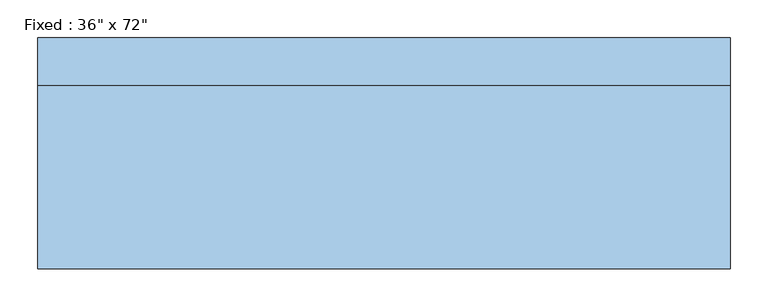
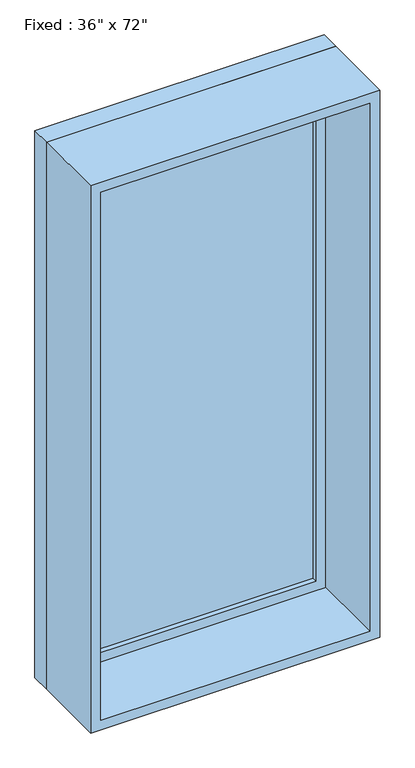
"""IFC4 building model written with IfcOpenShell, lengths in millimetres: window geometry."""

import ifcopenshell
import ifcopenshell.guid

model = None  # the IFC model being written
_history = None  # IfcOwnerHistory: only IFC2X3 demands one
_inside = {}  # id of a spatial element -> (the spatial element, [elements in it])
_under = {}  # id of a project, library or spatial element -> (it, [spatial elements below it])
_declared = {}  # id of a project -> (the project, [libraries it declares])
_typed = {}  # id of a type object -> (the type object, [elements of that type])
_made_of = {}  # id of a material, layer set ... -> (it, [elements and type objects made of it])


def new_model(schema):
    """Start an empty IFC model of exactly this schema.

    Asked for "IFC4X3", IfcOpenShell would pick the latest addendum, in which some entities
    have other attributes; the version numbers below select the first issue.
    IFC2X3 requires an IfcOwnerHistory on every rooted entity: one is made here for all.
    """
    global model, _history
    if schema == "IFC4X3":
        model = ifcopenshell.file(schema_version=(4, 3, 0, 0))
    else:
        model = ifcopenshell.file(schema=schema)
    _inside.clear()
    _under.clear()
    _declared.clear()
    _typed.clear()
    _made_of.clear()
    _history = None
    if model.schema == "IFC2X3":
        org = make("IfcOrganization", Name="unknown")
        user = make(
            "IfcPersonAndOrganization",
            ThePerson=make("IfcPerson", FamilyName="unknown"),
            TheOrganization=org,
        )
        app = make(
            "IfcApplication",
            ApplicationDeveloper=org,
            Version="unknown",
            ApplicationFullName="unknown",
            ApplicationIdentifier="unknown",
        )
        _history = make(
            "IfcOwnerHistory",
            OwningUser=user,
            OwningApplication=app,
            ChangeAction="ADDED",
            CreationDate=0,
        )
    return model


def make(cls, **values):
    """One entity of the class cls with the attributes given. An attribute that is None is left unset."""
    return model.create_entity(
        cls, **{name: value for name, value in values.items() if value is not None}
    )


def rooted(cls, **values):
    """An entity with a GlobalId (a new one), such as an element, a storey or a relation."""
    return make(cls, GlobalId=ifcopenshell.guid.new(), OwnerHistory=_history, **values)


def si_unit(unit_type, name, prefix=None):
    """IfcSIUnit, for example si_unit("LENGTHUNIT", "METRE", prefix="MILLI")."""
    return make("IfcSIUnit", UnitType=unit_type, Prefix=prefix, Name=name)


def assignment(units):
    """IfcUnitAssignment: the units of a project."""
    return None if units is None else make("IfcUnitAssignment", Units=units)


def point(xyz):
    """IfcCartesianPoint."""
    return None if xyz is None else make("IfcCartesianPoint", Coordinates=xyz)


def direction(xyz):
    """IfcDirection."""
    return None if xyz is None else make("IfcDirection", DirectionRatios=xyz)


def frame(location, z_axis=None, x_axis=None):
    """IfcAxis2Placement3D, a coordinate frame: its origin and axes. An axis left out is left unset."""
    return make(
        "IfcAxis2Placement3D",
        Location=point(location),
        Axis=direction(z_axis),
        RefDirection=direction(x_axis),
    )


def origin():
    """The frame at (0, 0, 0) with its axes left unset."""
    return frame((0.0, 0.0, 0.0))


def place(relative_to, where):
    """IfcLocalPlacement: puts the frame where relative to a parent placement (None: the world)."""
    return make(
        "IfcLocalPlacement", PlacementRelTo=relative_to, RelativePlacement=where
    )


def context(
    kind, dimensions, precision=None, world=None, true_north=None, identifier=None
):
    """IfcGeometricRepresentationContext, for example the 3D "Model" context."""
    return make(
        "IfcGeometricRepresentationContext",
        ContextIdentifier=identifier,
        ContextType=kind,
        CoordinateSpaceDimension=dimensions,
        Precision=precision,
        WorldCoordinateSystem=world,
        TrueNorth=true_north,
    )


def project(units=None, contexts=None):
    """IfcProject with its units and contexts."""
    return rooted(
        "IfcProject",
        Name="project",
        RepresentationContexts=contexts,
        UnitsInContext=assignment(units),
    )


def spatial(cls, under=None, at=None, **own):
    """A site, building, storey or space (cls), placed at a placement, below another one or the project."""
    s = rooted(cls, ObjectPlacement=at, **own)
    if under is not None:
        _under.setdefault(under.id(), (under, []))[1].append(s)
    return s


def polyline(points):
    """IfcPolyline through the points."""
    return make("IfcPolyline", Points=[point(p) for p in points])


def outline(outer, holes=None, kind="AREA"):
    """IfcArbitraryClosedProfileDef: a profile drawn as a closed curve; with holes, ...WithVoids."""
    if holes is None:
        return make("IfcArbitraryClosedProfileDef", ProfileType=kind, OuterCurve=outer)
    return make(
        "IfcArbitraryProfileDefWithVoids",
        ProfileType=kind,
        OuterCurve=outer,
        InnerCurves=holes,
    )


def extrude(swept, where, along, depth):
    """IfcExtrudedAreaSolid: the profile swept, set in the frame where, extruded along a direction by depth."""
    return make(
        "IfcExtrudedAreaSolid",
        SweptArea=swept,
        Position=where,
        ExtrudedDirection=direction(along),
        Depth=depth,
    )


def shape(context_of_items, identifier, shape_type, items):
    """IfcShapeRepresentation: the items that make up one representation, for example the "Body"."""
    return make(
        "IfcShapeRepresentation",
        ContextOfItems=context_of_items,
        RepresentationIdentifier=identifier,
        RepresentationType=shape_type,
        Items=items,
    )


def source(mapping_origin, context_of_items, identifier, shape_type, items):
    """IfcRepresentationMap: a shape defined once, which mapped items show again and again."""
    return make(
        "IfcRepresentationMap",
        MappingOrigin=mapping_origin,
        MappedRepresentation=shape(context_of_items, identifier, shape_type, items),
    )


def transform(
    local_origin,
    x_axis=None,
    y_axis=None,
    z_axis=None,
    scale=None,
    scale2=None,
    scale3=None,
    uniform=True,
):
    """IfcCartesianTransformationOperator3D, or its non-uniform kind. x_axis, y_axis, z_axis: its Axis1, 2, 3."""
    if uniform:
        return make(
            "IfcCartesianTransformationOperator3D",
            Axis1=direction(x_axis),
            Axis2=direction(y_axis),
            LocalOrigin=point(local_origin),
            Scale=scale,
            Axis3=direction(z_axis),
        )
    return make(
        "IfcCartesianTransformationOperator3DnonUniform",
        Axis1=direction(x_axis),
        Axis2=direction(y_axis),
        LocalOrigin=point(local_origin),
        Scale=scale,
        Axis3=direction(z_axis),
        Scale2=scale2,
        Scale3=scale3,
    )


def mapped(mapping_source, mapping_target):
    """IfcMappedItem: shows the shape of a source again, moved by a transform."""
    return make(
        "IfcMappedItem", MappingSource=mapping_source, MappingTarget=mapping_target
    )


def made_of(thing, what):
    """Note that an element or type object is made of a material, layer set ...; save() writes the relation."""
    if what is not None:
        _made_of.setdefault(what.id(), (what, []))[1].append(thing)
    return thing


def element(
    cls,
    number,
    at=None,
    inside=None,
    cuts=None,
    type_object=None,
    material=None,
    context=None,
    identifier="Body",
    shape_type=None,
    held_by="IfcProductDefinitionShape",
    body=None,
    shapes=None,
    **own,
):
    """One element of the class cls, such as IfcWall. Its Tag is "e" and its number.

    at: its placement. inside: the storey or other place that contains it. cuts: it is an
    opening in that element (IfcRelVoidsElement). A single representation is given by context,
    identifier, shape_type and body (its items); several are given by shapes. held_by: the class
    of the entity that holds the representations. save() writes the other relations.
    """
    e = rooted(cls, Tag="e%d" % number, ObjectPlacement=at, **own)
    if body is not None:
        shapes = [shape(context, identifier, shape_type, body)]
    if shapes is not None:
        e.Representation = make(held_by, Representations=shapes)
    if inside is not None:
        _inside.setdefault(inside.id(), (inside, []))[1].append(e)
    if cuts is not None:
        rooted(
            "IfcRelVoidsElement", RelatingBuildingElement=cuts, RelatedOpeningElement=e
        )
    if type_object is not None:
        _typed.setdefault(type_object.id(), (type_object, []))[1].append(e)
    return made_of(e, material)


def aggregate(whole, parts):
    """IfcRelAggregates: a whole, such as a stair, and the parts it consists of."""
    return rooted("IfcRelAggregates", RelatingObject=whole, RelatedObjects=parts)


def save(model, path):
    """Write the relations noted so far, then the file.

    IfcRelAggregates (storeys below a building ...), IfcRelContainedInSpatialStructure (elements
    in a storey), IfcRelDefinesByType, IfcRelAssociatesMaterial and IfcRelDeclares: one each for
    every whole, place, type object, material and project.
    """
    for whole, parts in _under.values():
        aggregate(whole, parts)
    for where, things in _inside.values():
        rooted(
            "IfcRelContainedInSpatialStructure",
            RelatedElements=things,
            RelatingStructure=where,
        )
    for kind, things in _typed.values():
        rooted("IfcRelDefinesByType", RelatedObjects=things, RelatingType=kind)
    for what, things in _made_of.values():
        rooted("IfcRelAssociatesMaterial", RelatedObjects=things, RelatingMaterial=what)
    for by, libraries in _declared.values():
        rooted("IfcRelDeclares", RelatingContext=by, RelatedDefinitions=libraries)
    model.write(path)


def window_c524ad49(model_context):
    return source(origin(), model_context, "Body", "SweptSolid", [
        extrude(outline(polyline([(355.6, 104.775), (-431.8, 104.775), (-431.8, 117.475), (355.6, 117.475), (355.6, 104.775)])), frame((0.0, 0.0, 368.3), z_axis=(0.0, 0.0, 1.0), x_axis=(1.0, 0.0, 0.0)), (0.0, 0.0, 1.0), 1701.8),
        extrude(outline(polyline([(2114.55, -476.25), (323.85, -476.25), (323.85, 400.05), (2114.55, 400.05), (2114.55, -476.25)]), holes=[polyline([(2070.1, -431.8), (2070.1, 355.6), (368.3, 355.6), (368.3, -431.8), (2070.1, -431.8)])]), frame((0.0, 88.9, 0.0), z_axis=(0.0, 1.0, 0.0), x_axis=(0.0, 0.0, 1.0)), (0.0, 0.0, 1.0), 44.45),
        extrude(outline(polyline([(2133.6, -495.3), (304.8, -495.3), (304.8, 419.1), (2133.6, 419.1), (2133.6, -495.3)]), holes=[polyline([(2101.85, -463.55), (2101.85, 387.35), (336.55, 387.35), (336.55, -463.55), (2101.85, -463.55)])]), frame((0.0, -152.4, 0.0), z_axis=(0.0, 1.0, 0.0), x_axis=(0.0, 0.0, 1.0)), (0.0, 0.0, 1.0), 241.3),
        extrude(outline(polyline([(2133.6, 419.1), (2133.6, -495.3), (304.8, -495.3), (304.8, 419.1), (2133.6, 419.1)]), holes=[polyline([(2114.55, 400.05), (323.85, 400.05), (323.85, -476.25), (2114.55, -476.25), (2114.55, 400.05)])]), frame((0.0, 88.9, 0.0), z_axis=(0.0, 1.0, 0.0), x_axis=(0.0, 0.0, 1.0)), (0.0, 0.0, 1.0), 63.5),
    ])


if __name__ == "__main__":
    model = new_model("IFC4")
    model_context = context("Model", 3, world=origin())
    ifc_project = project(units=[si_unit("LENGTHUNIT", "METRE", prefix="MILLI")], contexts=[model_context])
    site = spatial("IfcSite", under=ifc_project)
    building = spatial("IfcBuilding", under=site)
    placement = place(None, origin())
    window_shape = window_c524ad49(model_context)
    element("IfcWindow", 1, ObjectType="Fixed : 36\" x 72\"", at=placement, inside=building, context=model_context, shape_type="MappedRepresentation", body=[
        mapped(window_shape, transform((0.0, 0.0, 0.0), x_axis=(1.0, 0.0, 0.0), y_axis=(0.0, 1.0, 0.0), z_axis=(0.0, 0.0, 1.0))),
    ])
    save(model, "model.ifc")

# Revit data of these elements
# Type "Fixed : 36\" x 72\""
#   Type Mark = "18"
#   Construction Type Id = "GSP4R"
#   Assembly Code = "B2020100"
#   Analytic Construction = "1/8 in Pilkington single glazing"
#   Visual Light Transmittance = 0.9
#   Solar Heat Gain Coefficient = 0.78
#   Heat Transfer Coefficient (U) = 0.6496 BTU/(h·ft²·°F)
#   Height = 6' - 0"
#   Default Sill Height = 1' - 0"
#   Width = 3' - 0"
#   Window Inset = 0' - 0 3/4"
#   Define Thermal Properties by = 1
#   Define Thermal Properties by = 1
#   Glass Pane Material = Glass
#   Sash Material = Sash
#   Wall Closure = (empty or 0)
# Element 1 (IfcWindow, "Fixed : 36\" x 72\"")
#   Materials on its faces: "Sash", "Glass"
# Materials
#   "Glass": class "Glass", colour RGB 0 0 255, transparency 0.75, Description = "Soda Lime Glass", Cost = 0
#   "Sash": class "Wood", colour RGB 224 178 126, transparency 0
